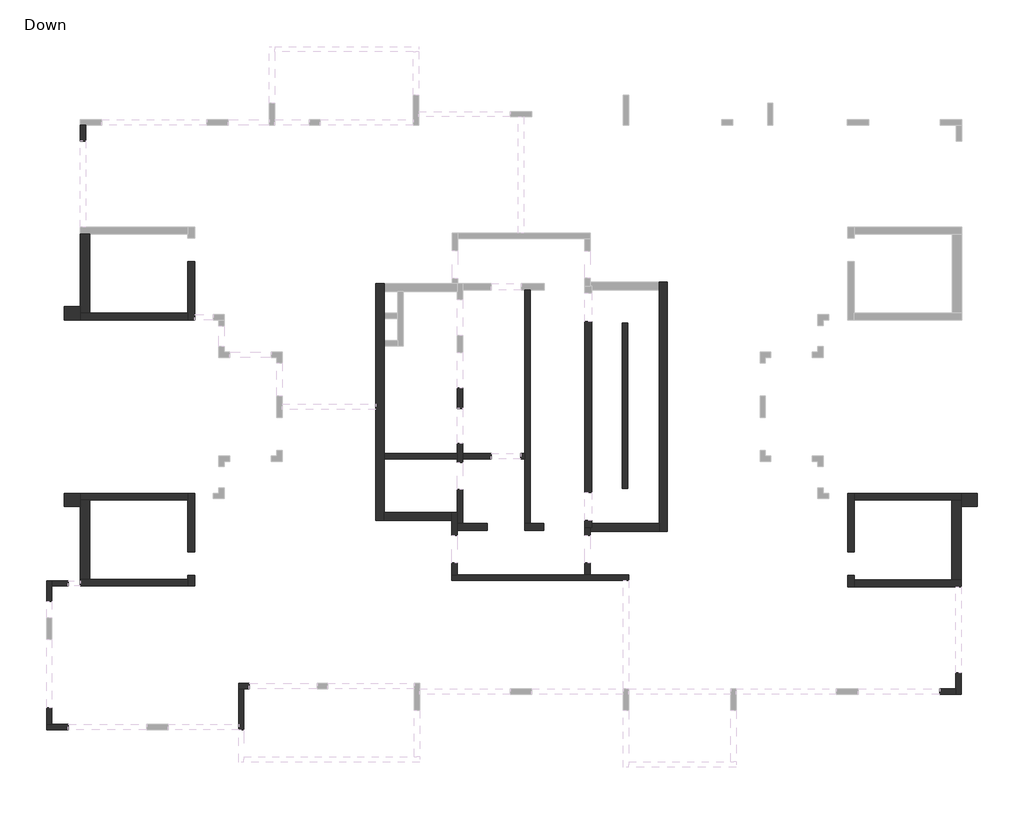
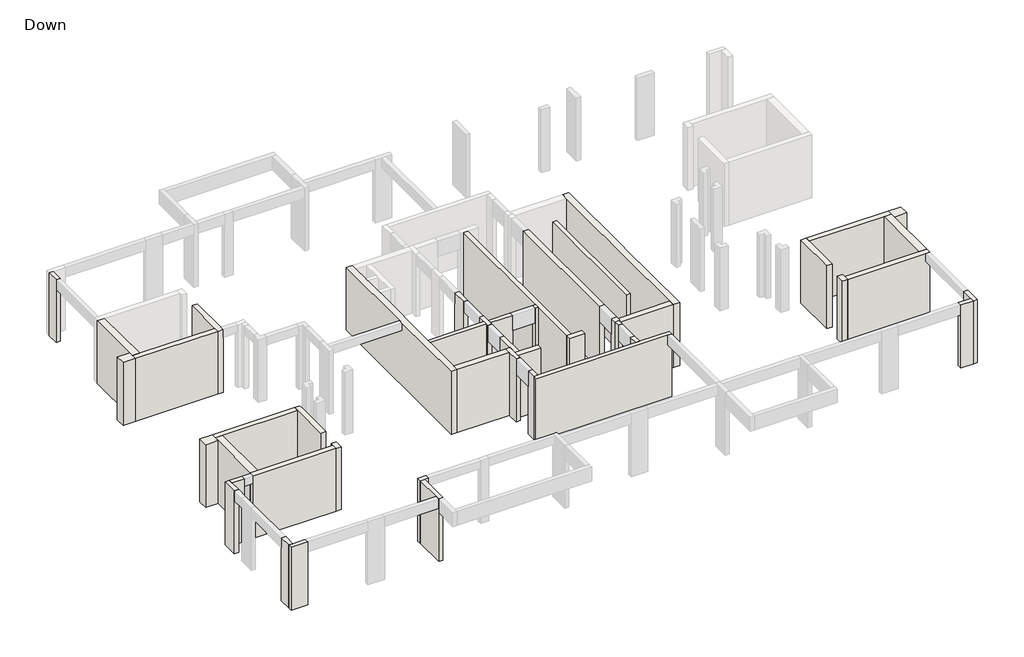
# One storey, part 1 of 3: 46 walls.
# Revit data of these elements (continued)
# Element 35 (IfcWall, "25") (continued)
#   Base Constraint = Down
#   Top Constraint = Typical Floor
#   Materials on its faces: "Concrete"
# Element 36 (IfcWall, "25")
#   Comments = ""
#   Mark = "W82"
#   SOFiSTiK_EdgeZones = "W84"
#   SOFiSTiK_AMG_Comments = ""
#   Top Offset = 0 cm
#   Base Offset = 0 cm
#   wall height = 320 cm
#   SOFiSTiK_AMG_Scheduled = yes
#   SOFiSTiK_AMG_Adjusted = yes
#   Phase Created = New Construction
#   Base Constraint = Down
#   Top Constraint = Typical Floor
#   Materials on its faces: "Concrete"
# Element 37 (IfcWall, "30")
#   Comments = ""
#   Mark = "W90"
#   SOFiSTiK_EdgeZones = "W92"
#   SOFiSTiK_AMG_Comments = ""
#   Top Offset = 0 cm
#   Base Offset = 0 cm
#   wall height = 320 cm
#   SOFiSTiK_AMG_Scheduled = yes
#   SOFiSTiK_AMG_Adjusted = yes
#   Phase Created = New Construction
#   Base Constraint = Down
#   Top Constraint = Typical Floor
#   Materials on its faces: "Concrete"
# Element 38 (IfcWall, "30")
#   Comments = ""
#   Mark = "W91"
#   SOFiSTiK_EdgeZones = "W93"
#   SOFiSTiK_AMG_Comments = ""
#   Top Offset = 0 cm
#   Base Offset = 0 cm
#   wall height = 320 cm
#   SOFiSTiK_AMG_Scheduled = yes
#   SOFiSTiK_AMG_Adjusted = yes
#   Phase Created = New Construction
#   Base Constraint = Down
#   Top Constraint = Typical Floor
#   Materials on its faces: "Concrete"
# Element 39 (IfcWall, "30")
#   Comments = ""
#   Mark = "W93"
#   SOFiSTiK_EdgeZones = "W95"
#   SOFiSTiK_AMG_Comments = ""
#   Top Offset = 0 cm
#   Base Offset = 0 cm
#   wall height = 320 cm
#   SOFiSTiK_AMG_Scheduled = yes
#   SOFiSTiK_AMG_Adjusted = yes
#   Phase Created = New Construction
#   Base Constraint = Down
#   Top Constraint = Typical Floor
#   Materials on its faces: "Concrete"
# Element 40 (IfcWall, "30")
#   Comments = ""
#   Mark = "W94"
#   SOFiSTiK_EdgeZones = "W96"
#   SOFiSTiK_AMG_Comments = ""
#   Top Offset = 0 cm
#   Base Offset = 0 cm
#   wall height = 320 cm
#   SOFiSTiK_AMG_Scheduled = yes
#   SOFiSTiK_AMG_Adjusted = yes
#   Phase Created = New Construction
#   Base Constraint = Down
#   Top Constraint = Typical Floor
#   Materials on its faces: "Concrete"
# Element 41 (IfcWall, "35")
#   Comments = ""
#   Mark = "W83"
#   SOFiSTiK_EdgeZones = "W85"
#   SOFiSTiK_AMG_Comments = ""
#   Top Offset = 0 cm
#   Base Offset = 0 cm
#   wall height = 320 cm
#   SOFiSTiK_AMG_Scheduled = yes
#   SOFiSTiK_AMG_Adjusted = yes
#   Phase Created = New Construction
#   Base Constraint = Down
#   Top Constraint = Typical Floor
#   Materials on its faces: "Concrete"
# Element 42 (IfcWall, "35")
#   Comments = ""
#   Mark = "W85"
#   SOFiSTiK_EdgeZones = "W87"
#   SOFiSTiK_AMG_Comments = ""
#   Top Offset = 0 cm
#   Base Offset = 0 cm
#   wall height = 320 cm
#   SOFiSTiK_AMG_Scheduled = yes
#   SOFiSTiK_AMG_Adjusted = yes
#   Phase Created = New Construction
#   Base Constraint = Down
#   Top Constraint = Typical Floor
#   Materials on its faces: "Concrete"
# Element 43 (IfcWall, "35")
#   Comments = ""
#   Mark = "W86"
#   SOFiSTiK_EdgeZones = "W88"
#   SOFiSTiK_AMG_Comments = ""
#   Top Offset = 0 cm
#   Base Offset = 0 cm
#   wall height = 320 cm
#   SOFiSTiK_AMG_Scheduled = yes
#   SOFiSTiK_AMG_Adjusted = yes
#   Phase Created = New Construction
#   Base Constraint = Down
#   Top Constraint = Typical Floor
#   Materials on its faces: "Concrete"
# Element 44 (IfcWall, "60")
#   Comments = ""
#   Mark = "W87"
#   SOFiSTiK_EdgeZones = "W89"
#   SOFiSTiK_AMG_Comments = ""
#   Top Offset = 0 cm
#   Base Offset = 0 cm
#   wall height = 320 cm
#   SOFiSTiK_AMG_Scheduled = yes
#   SOFiSTiK_AMG_Adjusted = yes
#   Phase Created = New Construction
#   Base Constraint = Down
#   Top Constraint = Typical Floor
#   Materials on its faces: "Concrete"
# Element 45 (IfcWall, "60")
#   Comments = ""
#   Mark = "W88"
#   SOFiSTiK_EdgeZones = "W90"
#   SOFiSTiK_AMG_Comments = ""
#   Top Offset = 0 cm
#   Base Offset = 0 cm
#   wall height = 320 cm
#   SOFiSTiK_AMG_Scheduled = yes
#   SOFiSTiK_AMG_Adjusted = yes
#   Phase Created = New Construction
#   Base Constraint = Down
#   Top Constraint = Typical Floor
#   Materials on its faces: "Concrete"
# Element 46 (IfcWall, "60")
#   Comments = ""
#   Mark = "W89"
#   SOFiSTiK_EdgeZones = "W91"
#   SOFiSTiK_AMG_Comments = ""
#   Top Offset = 0 cm
#   Base Offset = 0 cm
#   wall height = 320 cm
#   SOFiSTiK_AMG_Scheduled = yes
#   SOFiSTiK_AMG_Adjusted = yes
#   Phase Created = New Construction
#   Base Constraint = Down
#   Top Constraint = Typical Floor
#   Materials on its faces: "Concrete"
# Materials
#   "Concrete": class "Concrete", colour RGB 192 192 192, transparency 0, Keynote = "01000", Description = "Cast-in-place concrete", Cost = 0
